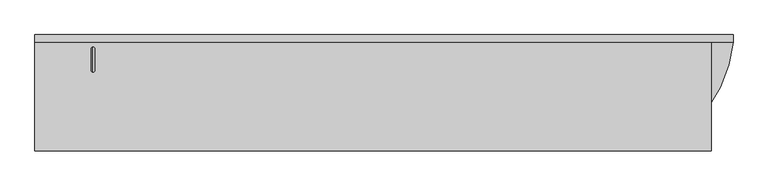
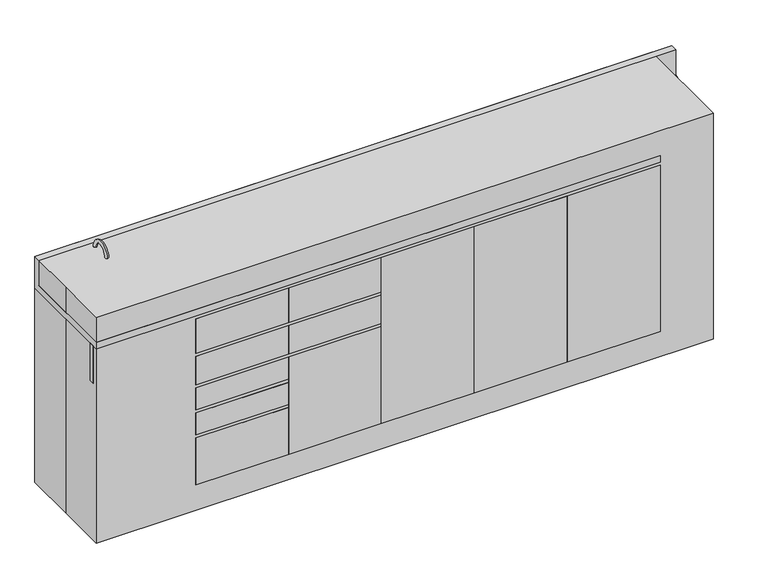
"""IFC4 building model written with IfcOpenShell, lengths in millimetres: proxy geometry, D0680 - Console, Accessory-Side, Dental Operatory-south sink-rounded : U0026 - Cabinet, Dental, Doctor's, Prosthodontic 2."""

import ifcopenshell
import ifcopenshell.guid

model = None  # the IFC model being written
_history = None  # IfcOwnerHistory: only IFC2X3 demands one
_inside = {}  # id of a spatial element -> (the spatial element, [elements in it])
_under = {}  # id of a project, library or spatial element -> (it, [spatial elements below it])
_declared = {}  # id of a project -> (the project, [libraries it declares])
_typed = {}  # id of a type object -> (the type object, [elements of that type])
_made_of = {}  # id of a material, layer set ... -> (it, [elements and type objects made of it])


def new_model(schema):
    """Start an empty IFC model of exactly this schema.

    Asked for "IFC4X3", IfcOpenShell would pick the latest addendum, in which some entities
    have other attributes; the version numbers below select the first issue.
    IFC2X3 requires an IfcOwnerHistory on every rooted entity: one is made here for all.
    """
    global model, _history
    if schema == "IFC4X3":
        model = ifcopenshell.file(schema_version=(4, 3, 0, 0))
    else:
        model = ifcopenshell.file(schema=schema)
    _inside.clear()
    _under.clear()
    _declared.clear()
    _typed.clear()
    _made_of.clear()
    _history = None
    if model.schema == "IFC2X3":
        org = make("IfcOrganization", Name="unknown")
        user = make(
            "IfcPersonAndOrganization",
            ThePerson=make("IfcPerson", FamilyName="unknown"),
            TheOrganization=org,
        )
        app = make(
            "IfcApplication",
            ApplicationDeveloper=org,
            Version="unknown",
            ApplicationFullName="unknown",
            ApplicationIdentifier="unknown",
        )
        _history = make(
            "IfcOwnerHistory",
            OwningUser=user,
            OwningApplication=app,
            ChangeAction="ADDED",
            CreationDate=0,
        )
    return model


def make(cls, **values):
    """One entity of the class cls with the attributes given. An attribute that is None is left unset."""
    return model.create_entity(
        cls, **{name: value for name, value in values.items() if value is not None}
    )


def rooted(cls, **values):
    """An entity with a GlobalId (a new one), such as an element, a storey or a relation."""
    return make(cls, GlobalId=ifcopenshell.guid.new(), OwnerHistory=_history, **values)


def si_unit(unit_type, name, prefix=None):
    """IfcSIUnit, for example si_unit("LENGTHUNIT", "METRE", prefix="MILLI")."""
    return make("IfcSIUnit", UnitType=unit_type, Prefix=prefix, Name=name)


def assignment(units):
    """IfcUnitAssignment: the units of a project."""
    return None if units is None else make("IfcUnitAssignment", Units=units)


def point(xyz):
    """IfcCartesianPoint."""
    return None if xyz is None else make("IfcCartesianPoint", Coordinates=xyz)


def direction(xyz):
    """IfcDirection."""
    return None if xyz is None else make("IfcDirection", DirectionRatios=xyz)


def frame(location, z_axis=None, x_axis=None):
    """IfcAxis2Placement3D, a coordinate frame: its origin and axes. An axis left out is left unset."""
    return make(
        "IfcAxis2Placement3D",
        Location=point(location),
        Axis=direction(z_axis),
        RefDirection=direction(x_axis),
    )


def frame_2d(location, x_axis=None):
    """IfcAxis2Placement2D, a coordinate frame in the plane: its origin and x axis."""
    return make(
        "IfcAxis2Placement2D", Location=point(location), RefDirection=direction(x_axis)
    )


def origin():
    """The frame at (0, 0, 0) with its axes left unset."""
    return frame((0.0, 0.0, 0.0))


def origin_with_axes():
    """The frame at (0, 0, 0) with the z axis (0, 0, 1) and the x axis (1, 0, 0) written out."""
    return frame((0.0, 0.0, 0.0), z_axis=(0.0, 0.0, 1.0), x_axis=(1.0, 0.0, 0.0))


def place(relative_to, where):
    """IfcLocalPlacement: puts the frame where relative to a parent placement (None: the world)."""
    return make(
        "IfcLocalPlacement", PlacementRelTo=relative_to, RelativePlacement=where
    )


def context(
    kind, dimensions, precision=None, world=None, true_north=None, identifier=None
):
    """IfcGeometricRepresentationContext, for example the 3D "Model" context."""
    return make(
        "IfcGeometricRepresentationContext",
        ContextIdentifier=identifier,
        ContextType=kind,
        CoordinateSpaceDimension=dimensions,
        Precision=precision,
        WorldCoordinateSystem=world,
        TrueNorth=true_north,
    )


def project(units=None, contexts=None):
    """IfcProject with its units and contexts."""
    return rooted(
        "IfcProject",
        Name="project",
        RepresentationContexts=contexts,
        UnitsInContext=assignment(units),
    )


def spatial(cls, under=None, at=None, **own):
    """A site, building, storey or space (cls), placed at a placement, below another one or the project."""
    s = rooted(cls, ObjectPlacement=at, **own)
    if under is not None:
        _under.setdefault(under.id(), (under, []))[1].append(s)
    return s


def polyline(points):
    """IfcPolyline through the points."""
    return make("IfcPolyline", Points=[point(p) for p in points])


def circle_curve(where, radius):
    """IfcCircle in the frame where."""
    return make("IfcCircle", Position=where, Radius=radius)


def ellipse_curve(where, semi_axis1, semi_axis2):
    """IfcEllipse in the frame where."""
    return make(
        "IfcEllipse", Position=where, SemiAxis1=semi_axis1, SemiAxis2=semi_axis2
    )


def trimmed(basis, trim1, trim2, sense, master):
    """IfcTrimmedCurve: the piece of a basis curve between two trims."""
    return make(
        "IfcTrimmedCurve",
        BasisCurve=basis,
        Trim1=trim1,
        Trim2=trim2,
        SenseAgreement=sense,
        MasterRepresentation=master,
    )


def segment(curve, same_sense, transition):
    """IfcCompositeCurveSegment."""
    return make(
        "IfcCompositeCurveSegment",
        Transition=transition,
        SameSense=same_sense,
        ParentCurve=curve,
    )


def composite_curve(segments, self_intersect=None):
    """IfcCompositeCurve: segments joined end to end."""
    return make("IfcCompositeCurve", Segments=segments, SelfIntersect=self_intersect)


def outline(outer, holes=None, kind="AREA"):
    """IfcArbitraryClosedProfileDef: a profile drawn as a closed curve; with holes, ...WithVoids."""
    if holes is None:
        return make("IfcArbitraryClosedProfileDef", ProfileType=kind, OuterCurve=outer)
    return make(
        "IfcArbitraryProfileDefWithVoids",
        ProfileType=kind,
        OuterCurve=outer,
        InnerCurves=holes,
    )


def extrude(swept, where, along, depth):
    """IfcExtrudedAreaSolid: the profile swept, set in the frame where, extruded along a direction by depth."""
    return make(
        "IfcExtrudedAreaSolid",
        SweptArea=swept,
        Position=where,
        ExtrudedDirection=direction(along),
        Depth=depth,
    )


def shape(context_of_items, identifier, shape_type, items):
    """IfcShapeRepresentation: the items that make up one representation, for example the "Body"."""
    return make(
        "IfcShapeRepresentation",
        ContextOfItems=context_of_items,
        RepresentationIdentifier=identifier,
        RepresentationType=shape_type,
        Items=items,
    )


def source(mapping_origin, context_of_items, identifier, shape_type, items):
    """IfcRepresentationMap: a shape defined once, which mapped items show again and again."""
    return make(
        "IfcRepresentationMap",
        MappingOrigin=mapping_origin,
        MappedRepresentation=shape(context_of_items, identifier, shape_type, items),
    )


def transform(
    local_origin,
    x_axis=None,
    y_axis=None,
    z_axis=None,
    scale=None,
    scale2=None,
    scale3=None,
    uniform=True,
):
    """IfcCartesianTransformationOperator3D, or its non-uniform kind. x_axis, y_axis, z_axis: its Axis1, 2, 3."""
    if uniform:
        return make(
            "IfcCartesianTransformationOperator3D",
            Axis1=direction(x_axis),
            Axis2=direction(y_axis),
            LocalOrigin=point(local_origin),
            Scale=scale,
            Axis3=direction(z_axis),
        )
    return make(
        "IfcCartesianTransformationOperator3DnonUniform",
        Axis1=direction(x_axis),
        Axis2=direction(y_axis),
        LocalOrigin=point(local_origin),
        Scale=scale,
        Axis3=direction(z_axis),
        Scale2=scale2,
        Scale3=scale3,
    )


def mapped(mapping_source, mapping_target):
    """IfcMappedItem: shows the shape of a source again, moved by a transform."""
    return make(
        "IfcMappedItem", MappingSource=mapping_source, MappingTarget=mapping_target
    )


def made_of(thing, what):
    """Note that an element or type object is made of a material, layer set ...; save() writes the relation."""
    if what is not None:
        _made_of.setdefault(what.id(), (what, []))[1].append(thing)
    return thing


def element(
    cls,
    number,
    at=None,
    inside=None,
    cuts=None,
    type_object=None,
    material=None,
    context=None,
    identifier="Body",
    shape_type=None,
    held_by="IfcProductDefinitionShape",
    body=None,
    shapes=None,
    **own,
):
    """One element of the class cls, such as IfcWall. Its Tag is "e" and its number.

    at: its placement. inside: the storey or other place that contains it. cuts: it is an
    opening in that element (IfcRelVoidsElement). A single representation is given by context,
    identifier, shape_type and body (its items); several are given by shapes. held_by: the class
    of the entity that holds the representations. save() writes the other relations.
    """
    e = rooted(cls, Tag="e%d" % number, ObjectPlacement=at, **own)
    if body is not None:
        shapes = [shape(context, identifier, shape_type, body)]
    if shapes is not None:
        e.Representation = make(held_by, Representations=shapes)
    if inside is not None:
        _inside.setdefault(inside.id(), (inside, []))[1].append(e)
    if cuts is not None:
        rooted(
            "IfcRelVoidsElement", RelatingBuildingElement=cuts, RelatedOpeningElement=e
        )
    if type_object is not None:
        _typed.setdefault(type_object.id(), (type_object, []))[1].append(e)
    return made_of(e, material)


def aggregate(whole, parts):
    """IfcRelAggregates: a whole, such as a stair, and the parts it consists of."""
    return rooted("IfcRelAggregates", RelatingObject=whole, RelatedObjects=parts)


def save(model, path):
    """Write the relations noted so far, then the file.

    IfcRelAggregates (storeys below a building ...), IfcRelContainedInSpatialStructure (elements
    in a storey), IfcRelDefinesByType, IfcRelAssociatesMaterial and IfcRelDeclares: one each for
    every whole, place, type object, material and project.
    """
    for whole, parts in _under.values():
        aggregate(whole, parts)
    for where, things in _inside.values():
        rooted(
            "IfcRelContainedInSpatialStructure",
            RelatedElements=things,
            RelatingStructure=where,
        )
    for kind, things in _typed.values():
        rooted("IfcRelDefinesByType", RelatedObjects=things, RelatingType=kind)
    for what, things in _made_of.values():
        rooted("IfcRelAssociatesMaterial", RelatedObjects=things, RelatingMaterial=what)
    for by, libraries in _declared.values():
        rooted("IfcRelDeclares", RelatingContext=by, RelatedDefinitions=libraries)
    model.write(path)


def plane_surface(at):
    """IfcPlane: the flat surface through the origin of the frame at, square to its z axis."""
    return make("IfcPlane", Position=at)


def cylinder_surface(at, radius):
    """IfcCylindricalSurface: all points at the distance radius from the z axis of the frame at."""
    return make("IfcCylindricalSurface", Position=at, Radius=radius)


def revolved_surface(curve, axis_point, axis_direction):
    """IfcSurfaceOfRevolution: the curve turned about the line through axis_point along axis_direction."""
    return make(
        "IfcSurfaceOfRevolution",
        SweptCurve=make("IfcArbitraryOpenProfileDef", ProfileType="CURVE", Curve=curve),
        AxisPosition=make("IfcAxis1Placement", Location=point(axis_point), Axis=direction(axis_direction)),
    )


def advanced_brep(points, edges, surfaces, faces):
    """IfcAdvancedBrep: a solid bounded by faces that lie on surfaces and meet in shared edges.

    An edge is (start, end): straight between two places in points (the first is 0);
    or (start, end, curve); or (start, end, curve, False) where it runs against its curve.
    A face is (place in surfaces, loops), or (place, loops, False) where it looks against
    its surface's normal. A loop lists edges by number (the first is 1), with a minus sign
    where the edge is run from its end to its start. The first loop is the outer one.
    """
    corners = [point(p) for p in points]
    vertices = [make("IfcVertexPoint", VertexGeometry=c) for c in corners]
    made = []
    for start, end, *more in edges:
        made.append(
            make(
                "IfcEdgeCurve",
                EdgeStart=vertices[start],
                EdgeEnd=vertices[end],
                EdgeGeometry=more[0] if more else make("IfcPolyline", Points=[corners[start], corners[end]]),
                SameSense=more[1] if len(more) > 1 else True,
            )
        )
    hull = []
    for where, loops, *sense in faces:
        bounds = []
        for j, loop in enumerate(loops):
            ring = [make("IfcOrientedEdge", EdgeElement=made[abs(k) - 1], Orientation=k > 0) for k in loop]
            bounds.append(
                make(
                    "IfcFaceOuterBound" if j == 0 else "IfcFaceBound",
                    Bound=make("IfcEdgeLoop", EdgeList=ring),
                    Orientation=True,
                )
            )
        hull.append(make("IfcAdvancedFace", Bounds=bounds, FaceSurface=surfaces[where], SameSense=sense[0] if sense else True))
    return make("IfcAdvancedBrep", Outer=make("IfcClosedShell", CfsFaces=hull))


def specialty_equipment_783713db(model_context):
    return source(origin(), model_context, "Body", "SolidModel", [
        advanced_brep(
        [(-1014.0443585, -165.0080446, 787.3899582), (-1014.0443585, 139.7919554, 787.3899582), (-1014.0443585, 128.6794554, 787.3899582), (-1014.0443585, -153.8955446, 787.3899582), (-1014.0443585, 127.0919554, 785.8024582), (-1014.0443585, -152.3080446, 785.8024582), (-1014.0443585, 127.0919554, 730.25), (-1014.0443585, -152.3080446, 730.25), (-1014.0443585, -101.5080446, 679.45), (-1014.0443585, 76.2919554, 679.45), (-1014.0443585, -0.1899284, 679.45), (-1003.5461263, -12.6976148, 679.45), (-1014.0443585, -25.2053012, 679.45), (-1028.9461263, -12.6976148, 679.45), (-1014.0443585, -158.6580446, 676.275), (-1014.0443585, 133.4419554, 676.275), (-1014.0443585, 133.4419554, 784.0168572), (-1014.0443585, -158.6580446, 784.0168572), (-1014.0443585, 139.7919554, 784.0168572), (-1014.0443585, -165.0080446, 784.0168572), (-1014.0443585, -25.2053012, 676.275), (-1003.5461263, -12.6976148, 676.275), (-1014.0443585, -0.1899284, 676.275), (-1028.9461263, -12.6976148, 676.275)],
        [
            (0, 1, circle_curve(frame((-1014.0443585, -12.6080446, 787.3899582), z_axis=(0.0, 0.0, 1.0), x_axis=(0.0, 1.0, 0.0)), 152.4)),
            (1, 2),
            (2, 3, circle_curve(frame((-1014.0443585, -12.6080446, 787.3899582), z_axis=(0.0, 0.0, -1.0), x_axis=(0.0, 1.0, 0.0)), 141.2875)),
            (3, 0),
            (1, 0, circle_curve(frame((-1014.0443585, -12.6080446, 787.3899582), z_axis=(0.0, 0.0, 1.0), x_axis=(0.0, 1.0, 0.0)), 152.4)),
            (3, 2, circle_curve(frame((-1014.0443585, -12.6080446, 787.3899582), z_axis=(0.0, 0.0, -1.0), x_axis=(0.0, 1.0, 0.0)), 141.2875)),
            (2, 4, circle_curve(frame((-1014.0443585, 128.6794554, 785.8024582), z_axis=(1.0, 0.0, 0.0), x_axis=(0.0, 1.0, 0.0)), 1.5875)),
            (4, 5, circle_curve(frame((-1014.0443585, -12.6080446, 785.8024582), z_axis=(0.0, 0.0, -1.0), x_axis=(0.0, 1.0, 0.0)), 139.7)),
            (5, 3, circle_curve(frame((-1014.0443585, -153.8955446, 785.8024582), z_axis=(1.0, 0.0, 0.0), x_axis=(0.0, -1.0, 0.0)), 1.5875)),
            (5, 4, circle_curve(frame((-1014.0443585, -12.6080446, 785.8024582), z_axis=(0.0, 0.0, -1.0), x_axis=(0.0, 1.0, 0.0)), 139.7)),
            (4, 6),
            (6, 7, circle_curve(frame((-1014.0443585, -12.6080446, 730.25), z_axis=(0.0, 0.0, -1.0), x_axis=(0.0, 1.0, 0.0)), 139.7)),
            (7, 5),
            (7, 6, circle_curve(frame((-1014.0443585, -12.6080446, 730.25), z_axis=(0.0, 0.0, -1.0), x_axis=(0.0, 1.0, 0.0)), 139.7)),
            (8, 9, circle_curve(frame((-1014.0443585, -12.6080446, 679.45), z_axis=(0.0, 0.0, 1.0), x_axis=(0.0, 1.0, 0.0)), 88.9)),
            (9, 10),
            (10, 11, circle_curve(frame((-1016.2461263, -12.6976148, 679.45), z_axis=(0.0, 0.0, -1.0), x_axis=(-1.0, 0.0, 0.0)), 12.7)),
            (11, 12, circle_curve(frame((-1016.2461263, -12.6976148, 679.45), z_axis=(0.0, 0.0, -1.0), x_axis=(-1.0, 0.0, 0.0)), 12.7)),
            (12, 8),
            (9, 8, circle_curve(frame((-1014.0443585, -12.6080446, 679.45), z_axis=(0.0, 0.0, 1.0), x_axis=(0.0, 1.0, 0.0)), 88.9)),
            (12, 13, circle_curve(frame((-1016.2461263, -12.6976148, 679.45), z_axis=(0.0, 0.0, -1.0), x_axis=(-1.0, 0.0, 0.0)), 12.7)),
            (13, 10, circle_curve(frame((-1016.2461263, -12.6976148, 679.45), z_axis=(0.0, 0.0, -1.0), x_axis=(-1.0, 0.0, 0.0)), 12.7)),
            (14, 15, circle_curve(frame((-1014.0443585, -12.6080446, 676.275), z_axis=(0.0, 0.0, 1.0), x_axis=(0.0, 1.0, 0.0)), 146.05)),
            (15, 16),
            (16, 17, circle_curve(frame((-1014.0443585, -12.6080446, 784.0168572), z_axis=(0.0, 0.0, -1.0), x_axis=(0.0, 1.0, 0.0)), 146.05)),
            (17, 14),
            (15, 14, circle_curve(frame((-1014.0443585, -12.6080446, 676.275), z_axis=(0.0, 0.0, 1.0), x_axis=(0.0, 1.0, 0.0)), 146.05)),
            (17, 16, circle_curve(frame((-1014.0443585, -12.6080446, 784.0168572), z_axis=(0.0, 0.0, -1.0), x_axis=(0.0, 1.0, 0.0)), 146.05)),
            (16, 18),
            (18, 19, circle_curve(frame((-1014.0443585, -12.6080446, 784.0168572), z_axis=(0.0, 0.0, -1.0), x_axis=(0.0, 1.0, 0.0)), 152.4)),
            (19, 17),
            (19, 18, circle_curve(frame((-1014.0443585, -12.6080446, 784.0168572), z_axis=(0.0, 0.0, -1.0), x_axis=(0.0, 1.0, 0.0)), 152.4)),
            (0, 19),
            (18, 1),
            (14, 20),
            (20, 21, circle_curve(frame((-1016.2461263, -12.6976148, 676.275), z_axis=(0.0, 0.0, 1.0), x_axis=(-1.0, 0.0, 0.0)), 12.7)),
            (21, 22, circle_curve(frame((-1016.2461263, -12.6976148, 676.275), z_axis=(0.0, 0.0, 1.0), x_axis=(-1.0, 0.0, 0.0)), 12.7)),
            (22, 15),
            (22, 23, circle_curve(frame((-1016.2461263, -12.6976148, 676.275), z_axis=(0.0, 0.0, 1.0), x_axis=(-1.0, 0.0, 0.0)), 12.7)),
            (23, 20, circle_curve(frame((-1016.2461263, -12.6976148, 676.275), z_axis=(0.0, 0.0, 1.0), x_axis=(-1.0, 0.0, 0.0)), 12.7)),
            (6, 9, circle_curve(frame((-1014.0443585, 76.2919554, 730.25), z_axis=(-1.0, 0.0, 0.0), x_axis=(0.0, 1.0, 0.0)), 50.8)),
            (8, 7, circle_curve(frame((-1014.0443585, -101.5080446, 730.25), z_axis=(-1.0, 0.0, 0.0), x_axis=(0.0, -1.0, 0.0)), 50.8)),
            (23, 13),
            (11, 21),
        ],
        [
            plane_surface(frame((-1014.0443585, -12.6080446, 787.3899582), z_axis=(0.0, 0.0, 1.0), x_axis=(0.0, 1.0, 0.0))),
            revolved_surface(trimmed(ellipse_curve(frame((-1014.0443585, 128.6794554, 785.8024582), z_axis=(-1.0, 0.0, 0.0), x_axis=(0.0, 1.0, 0.0)), 1.5875, 1.5875), [point((-1014.0443585, 127.0919554, 785.8024582))], [point((-1014.0443585, 128.6794554, 787.3899582))], True, "CARTESIAN"), (-1014.0443585, -12.6080446, 787.4), (0.0, 0.0, -1.0)),
            revolved_surface(polyline([(-1014.0443585, 127.09195539999999, 730.25), (-1014.0443585, 127.09195539999999, 785.8024582)]), (-1014.0443585, -12.6080446, 787.4), (0.0, 0.0, -1.0)),
            plane_surface(frame((-1014.0443585, -12.6080446, 679.45), z_axis=(0.0, 0.0, 1.0), x_axis=(0.0, 1.0, 0.0))),
            cylinder_surface(frame((-1014.0443585, -12.6080446, 787.4), z_axis=(0.0, 0.0, -1.0), x_axis=(0.0, 1.0, 0.0)), 146.05),
            plane_surface(frame((-1014.0443585, -12.6080446, 784.0168572), z_axis=(0.0, 0.0, -1.0), x_axis=(0.0, 1.0, 0.0))),
            cylinder_surface(frame((-1014.0443585, -12.6080446, 787.4), z_axis=(0.0, 0.0, -1.0), x_axis=(0.0, 1.0, 0.0)), 152.4),
            plane_surface(frame((-1014.0443585, -12.6080446, 676.275), z_axis=(0.0, 0.0, -1.0), x_axis=(0.0, 1.0, 0.0))),
            revolved_surface(trimmed(ellipse_curve(frame((-1014.0443585, 76.2919554, 730.25), z_axis=(1.0, 0.0, 0.0), x_axis=(0.0, 1.0, 0.0)), 50.8, 50.8), [point((-1014.0443585, 76.2919554, 679.45))], [point((-1014.0443585, 127.0919554, 730.25))], True, "CARTESIAN"), (-1014.0443585, -12.6080446, 787.4), (0.0, 0.0, -1.0)),
            revolved_surface(polyline([(-1028.9461263, -12.6976148, 679.45), (-1028.9461263, -12.6976148, 676.275)]), (-1016.2461263, -12.6976148, 673.1), (0.0, 0.0, 1.0)),
        ],
        [
            (0, [[1, 2, 3, 4]]),
            (0, [[-2, 5, -4, 6]]),
            (1, [[-3, 7, 8, 9]]),
            (1, [[-6, -9, 10, -7]]),
            (2, [[-8, 11, 12, 13]]),
            (2, [[-10, -13, 14, -11]]),
            (3, [[15, 16, 17, 18, 19]]),
            (3, [[20, -19, 21, 22, -16]]),
            (4, [[23, 24, 25, 26]]),
            (4, [[-24, 27, -26, 28]]),
            (5, [[-25, 29, 30, 31]]),
            (5, [[-28, -31, 32, -29]]),
            (6, [[-1, 33, -30, 34]]),
            (6, [[-5, -34, -32, -33]]),
            (7, [[-23, 35, 36, 37, 38]]),
            (7, [[-27, -38, 39, 40, -35]]),
            (8, [[-12, 41, -15, 42]]),
            (8, [[-14, -42, -20, -41]]),
            (9, [[43, -21, -18, 44, -36, -40]]),
            (9, [[-43, -39, -37, -44, -17, -22]]),
        ],
    ),
        extrude(outline(polyline([(-1219.2, -184.15), (-1219.2, -165.1), (-850.9, -165.1), (-850.9, -184.15), (-1219.2, -184.15)])), frame((0.0, 0.0, 635.0), z_axis=(0.0, 0.0, 1.0), x_axis=(1.0, 0.0, 0.0)), (0.0, 0.0, 1.0), 152.4),
        extrude(outline(polyline([(-184.15, 101.6), (-203.2, 101.6), (-203.2, 774.4822891), (-193.675, 774.4822891), (-193.675, 787.2846899), (-184.15, 787.2846899), (-184.15, 101.6)])), frame((584.2, 0.0, 0.0), z_axis=(1.0, 0.0, 0.0), x_axis=(0.0, 1.0, 0.0)), (0.0, 0.0, 1.0), 355.6),
        extrude(outline(polyline([(-184.15, 101.6), (-203.2, 101.6), (-203.2, 774.7), (-193.675, 774.7), (-193.675, 787.4), (-184.15, 787.4), (-184.15, 101.6)])), frame((228.6, 0.0, 0.0), z_axis=(1.0, 0.0, 0.0), x_axis=(0.0, 1.0, 0.0)), (0.0, 0.0, 1.0), 355.6),
        extrude(outline(polyline([(-184.15, 101.6), (-203.2, 101.6), (-203.2, 774.7), (-193.675, 774.7), (-193.675, 787.4), (-184.15, 787.4), (-184.15, 101.6)])), frame((-127.0, 0.0, 0.0), z_axis=(1.0, 0.0, 0.0), x_axis=(0.0, 1.0, 0.0)), (0.0, 0.0, 1.0), 355.6),
        extrude(outline(polyline([(-193.675, 774.7), (-193.675, 787.4), (-184.15, 787.4), (-184.15, 635.0), (-203.2, 635.0), (-203.2, 774.7), (-193.675, 774.7)])), frame((-482.6, 0.0, 0.0), z_axis=(1.0, 0.0, 0.0), x_axis=(0.0, 1.0, 0.0)), (0.0, 0.0, 1.0), 355.6),
        extrude(outline(polyline([(-193.675, 622.9156171), (-193.675, 635.0), (-184.15, 635.0), (-184.15, 508.0524006), (-203.2, 508.0524006), (-203.2, 622.9156171), (-193.675, 622.9156171)])), frame((-482.6, 0.0, 0.0), z_axis=(1.0, 0.0, 0.0), x_axis=(0.0, 1.0, 0.0)), (0.0, 0.0, 1.0), 355.6),
        extrude(outline(polyline([(-193.675, 495.2120809), (-193.675, 508.0517033), (-184.15, 508.0517033), (-184.15, 101.6), (-203.2, 101.6), (-203.2, 495.2120809), (-193.675, 495.2120809)])), frame((-482.6, 0.0, 0.0), z_axis=(1.0, 0.0, 0.0), x_axis=(0.0, 1.0, 0.0)), (0.0, 0.0, 1.0), 355.6),
        extrude(outline(composite_curve([segment(trimmed(circle_curve(frame_2d((-1053.7479232, 156.0133962)), 12.7), [point((-1041.0479232, 156.0133962))], [point((-1066.4479232, 156.0133962))], False, "CARTESIAN"), True, "CONTINUOUS"), segment(trimmed(circle_curve(frame_2d((-1053.7479232, 156.0133962)), 12.7), [point((-1066.4479232, 156.0133962))], [point((-1041.0479232, 156.0133962))], False, "CARTESIAN"), True, "CONTINUOUS")], self_intersect=False)), frame((0.0, 0.0, 812.8), z_axis=(0.0, 0.0, 1.0), x_axis=(1.0, 0.0, 0.0)), (0.0, 0.0, 1.0), 31.75),
        extrude(outline(composite_curve([segment(trimmed(circle_curve(frame_2d((-980.5384765, 156.0133962)), 12.7), [point((-967.8384765, 156.0133962))], [point((-993.2384765, 156.0133962))], False, "CARTESIAN"), True, "CONTINUOUS"), segment(trimmed(circle_curve(frame_2d((-980.5384765, 156.0133962)), 12.7), [point((-993.2384765, 156.0133962))], [point((-967.8384765, 156.0133962))], False, "CARTESIAN"), True, "CONTINUOUS")], self_intersect=False)), frame((0.0, 0.0, 812.8), z_axis=(0.0, 0.0, 1.0), x_axis=(1.0, 0.0, 0.0)), (0.0, 0.0, 1.0), 31.75),
        advanced_brep(
        [(-1016.415785, 148.0147812, 812.8), (-1016.415785, 160.7147812, 812.8), (-1016.415785, 160.7147812, 914.4), (-1016.415785, 148.0147812, 914.4), (-1016.415785, 84.5147812, 914.4), (-1016.415785, 71.8147812, 914.4)],
        [
            (0, 1, circle_curve(frame((-1016.415785, 154.3647812, 812.8), z_axis=(0.0, 0.0, -1.0), x_axis=(0.0, 1.0, 0.0)), 6.35)),
            (1, 0, circle_curve(frame((-1016.415785, 154.3647812, 812.8), z_axis=(0.0, 0.0, -1.0), x_axis=(0.0, 1.0, 0.0)), 6.35)),
            (1, 2),
            (2, 3, circle_curve(frame((-1016.415785, 154.3647812, 914.4), z_axis=(0.0, 0.0, -1.0), x_axis=(0.0, 1.0, 0.0)), 6.35)),
            (3, 0),
            (3, 2, circle_curve(frame((-1016.415785, 154.3647812, 914.4), z_axis=(0.0, 0.0, -1.0), x_axis=(0.0, 1.0, 0.0)), 6.35)),
            (4, 5, circle_curve(frame((-1016.415785, 78.1647812, 914.4), z_axis=(0.0, 0.0, -1.0), x_axis=(0.0, -1.0, 0.0)), 6.35)),
            (5, 4, circle_curve(frame((-1016.415785, 78.1647812, 914.4), z_axis=(0.0, 0.0, -1.0), x_axis=(0.0, -1.0, 0.0)), 6.35)),
            (4, 3, circle_curve(frame((-1016.415785, 116.2647812, 914.4), z_axis=(-1.0, 0.0, 0.0), x_axis=(0.0, 1.0, 0.0)), 31.75)),
            (2, 5, circle_curve(frame((-1016.415785, 116.2647812, 914.4), z_axis=(1.0, 0.0, 0.0), x_axis=(0.0, 1.0, 0.0)), 44.45)),
        ],
        [
            plane_surface(frame((-1104.9, 154.3647812, 812.8), z_axis=(0.0, 0.0, -1.0), x_axis=(-1.0, 0.0, 0.0))),
            cylinder_surface(frame((-1016.415785, 154.3647812, 812.8), z_axis=(0.0, 0.0, -1.0), x_axis=(0.0, 1.0, 0.0)), 6.35),
            plane_surface(frame((-1104.9, 78.1647812, 914.4), z_axis=(0.0, 0.0, -1.0), x_axis=(-1.0, 0.0, 0.0))),
            revolved_surface(trimmed(ellipse_curve(frame((-1016.415785, 154.3647812, 914.4), z_axis=(0.0, 0.0, -1.0), x_axis=(0.0, 1.0, 0.0)), 6.35, 6.35), [point((-1016.415785, 160.7147812, 914.4))], [point((-1016.415785, 148.0147812, 914.4))], True, "CARTESIAN"), (-1104.9, 116.2647812, 914.4), (1.0, 0.0, 0.0)),
            revolved_surface(trimmed(ellipse_curve(frame((-1016.415785, 154.3647812, 914.4), z_axis=(0.0, 0.0, -1.0), x_axis=(0.0, 1.0, 0.0)), 6.35, 6.35), [point((-1016.415785, 148.0147812, 914.4))], [point((-1016.415785, 160.7147812, 914.4))], True, "CARTESIAN"), (-1104.9, 116.2647812, 914.4), (1.0, 0.0, 0.0)),
        ],
        [
            (0, [[1, 2]]),
            (1, [[-2, 3, 4, 5]]),
            (1, [[-1, -5, 6, -3]]),
            (2, [[7, 8]]),
            (3, [[9, -4, 10, -7]]),
            (4, [[-10, -6, -9, -8]]),
        ],
    ),
        extrude(outline(polyline([(-193.675, 774.7), (-193.675, 787.4), (-184.15, 787.4), (-184.15, 635.0), (-203.2, 635.0), (-203.2, 774.7), (-193.675, 774.7)])), frame((-838.2, 0.0, 0.0), z_axis=(1.0, 0.0, 0.0), x_axis=(0.0, 1.0, 0.0)), (0.0, 0.0, 1.0), 355.6),
        extrude(outline(polyline([(-193.675, 622.9156171), (-193.675, 635.0), (-184.15, 635.0), (-184.15, 508.0), (-203.2, 508.0), (-203.2, 622.9156171), (-193.675, 622.9156171)])), frame((-838.2, 0.0, 0.0), z_axis=(1.0, 0.0, 0.0), x_axis=(0.0, 1.0, 0.0)), (0.0, 0.0, 1.0), 355.6),
        extrude(outline(polyline([(-193.675, 495.3), (-193.675, 508.0), (-184.15, 508.0), (-184.15, 406.4), (-203.2, 406.4), (-203.2, 495.3), (-193.675, 495.3)])), frame((-838.2, 0.0, 0.0), z_axis=(1.0, 0.0, 0.0), x_axis=(0.0, 1.0, 0.0)), (0.0, 0.0, 1.0), 355.6),
        extrude(outline(polyline([(-193.675, 393.7), (-193.675, 406.4), (-184.15, 406.4), (-184.15, 304.8), (-203.2, 304.8), (-203.2, 393.7), (-193.675, 393.7)])), frame((-838.2, 0.0, 0.0), z_axis=(1.0, 0.0, 0.0), x_axis=(0.0, 1.0, 0.0)), (0.0, 0.0, 1.0), 355.6),
        extrude(outline(polyline([(-193.675, 292.1), (-193.675, 304.8), (-184.15, 304.8), (-184.15, 101.6), (-203.2, 101.6), (-203.2, 292.1), (-193.675, 292.1)])), frame((-838.2, 0.0, 0.0), z_axis=(1.0, 0.0, 0.0), x_axis=(0.0, 1.0, 0.0)), (0.0, 0.0, 1.0), 355.6),
        advanced_brep(
        [(-1219.2, 177.8, 914.4), (-1219.2, 203.2, 914.4), (-1219.2, 203.2, 787.4), (-1219.2, -203.2, 787.4), (-1219.2, -203.2, 812.8), (-1219.2, 177.8, 812.8), (1219.2, 177.8, 812.8), (1219.2, 177.8, 863.6), (1219.2, 177.8, 914.4), (939.8, -203.2, 812.8), (-874.2071906, -12.5959993, 812.8), (-1153.6071906, -12.5959993, 812.8), (939.8, -203.2, 787.4), (1219.2, 203.2, 787.4), (1219.2, 177.8, 787.4), (-1153.6071906, -12.5959993, 787.4), (-874.2071906, -12.5959993, 787.4), (1219.2, 203.2, 914.4)],
        [
            (0, 1),
            (1, 2),
            (2, 3),
            (3, 4),
            (4, 5),
            (5, 0),
            (5, 6),
            (6, 7),
            (7, 8),
            (8, 0),
            (4, 9),
            (9, 6, circle_curve(frame((763.8405952, 218.7835635, 812.8), z_axis=(0.0, 0.0, 1.0), x_axis=(1.0, 0.0, 0.0)), 457.2)),
            (10, 11, circle_curve(frame((-1013.9071906, -12.5959993, 812.8), z_axis=(0.0, 0.0, -1.0), x_axis=(-1.0, 0.0, 0.0)), 139.7)),
            (11, 10, circle_curve(frame((-1013.9071906, -12.5959993, 812.8), z_axis=(0.0, 0.0, -1.0), x_axis=(-1.0, 0.0, 0.0)), 139.7)),
            (3, 12),
            (12, 9),
            (2, 13),
            (13, 14),
            (14, 12, circle_curve(frame((763.8405952, 218.7835635, 787.4), z_axis=(0.0, 0.0, -1.0), x_axis=(1.0, 0.0, 0.0)), 457.2)),
            (15, 16, circle_curve(frame((-1013.9071906, -12.5959993, 787.4), z_axis=(0.0, 0.0, 1.0), x_axis=(-1.0, 0.0, 0.0)), 139.7)),
            (16, 15, circle_curve(frame((-1013.9071906, -12.5959993, 787.4), z_axis=(0.0, 0.0, 1.0), x_axis=(-1.0, 0.0, 0.0)), 139.7)),
            (17, 13),
            (1, 17),
            (8, 17),
            (15, 11),
            (10, 16),
            (6, 14),
        ],
        [
            plane_surface(frame((-1219.2, 177.8, 812.8), z_axis=(-1.0, 0.0, 0.0), x_axis=(0.0, 0.0, 1.0))),
            plane_surface(frame((1219.2, 177.8, 914.4), z_axis=(0.0, -1.0, 0.0), x_axis=(-1.0, 0.0, 0.0))),
            plane_surface(frame((1219.2, 177.8, 812.8), z_axis=(0.0, 0.0, 1.0), x_axis=(-1.0, 0.0, 0.0))),
            plane_surface(frame((1219.2, -203.2, 812.8), z_axis=(0.0, -1.0, 0.0), x_axis=(-1.0, 0.0, 0.0))),
            plane_surface(frame((1219.2, -203.2, 787.4), z_axis=(0.0, 0.0, -1.0), x_axis=(-1.0, 0.0, 0.0))),
            plane_surface(frame((1219.2, 203.2, 787.4), z_axis=(0.0, 1.0, 0.0), x_axis=(-1.0, 0.0, 0.0))),
            plane_surface(frame((1219.2, 203.2, 914.4), z_axis=(0.0, 0.0, 1.0), x_axis=(-1.0, 0.0, 0.0))),
            revolved_surface(polyline([(-1153.6071906, -12.5959993, 812.8), (-1153.6071906, -12.5959993, 787.4)]), (-1013.9071906, -12.5959993, 768.35), (0.0, 0.0, 1.0)),
            plane_surface(frame((1219.2, 177.8, 812.8), z_axis=(1.0, 0.0, 0.0), x_axis=(0.0, 0.0, -1.0))),
            cylinder_surface(frame((763.8405952, 218.7835635, 736.6), z_axis=(0.0, 0.0, -1.0), x_axis=(1.0, 0.0, 0.0)), 457.2),
        ],
        [
            (0, [[1, 2, 3, 4, 5, 6]]),
            (1, [[-6, 7, 8, 9, 10]]),
            (2, [[-5, 11, 12, -7], [13, 14]]),
            (3, [[-4, 15, 16, -11]]),
            (4, [[-3, 17, 18, 19, -15], [20, 21]]),
            (5, [[22, -17, -2, 23]]),
            (6, [[24, -23, -1, -10]]),
            (7, [[25, -13, 26, -20]]),
            (7, [[-25, -21, -26, -14]]),
            (8, [[-22, -24, -9, -8, 27, -18]]),
            (9, [[-27, -12, -16, -19]]),
        ],
    ),
        extrude(outline(polyline([(-1219.2, 203.2), (1143.0, 203.2), (1143.0, -203.2), (-1219.2, -203.2), (-1219.2, 0.0), (-1219.2, 203.2)])), origin_with_axes(), (0.0, 0.0, 1.0), 914.4),
        extrude(outline(polyline([(184.15, 785.890324), (184.15, 0.0), (-165.1, 0.0), (-165.1, 101.6), (-184.15, 101.6), (-184.15, 785.890324), (184.15, 785.890324)])), frame((939.8, 0.0, 0.0), z_axis=(1.0, 0.0, 0.0), x_axis=(0.0, 1.0, 0.0)), (0.0, 0.0, 1.0), 12.7),
        extrude(outline(polyline([(1199.3554733, 184.15), (-850.9, 184.15), (-850.9, 203.2), (1199.3554733, 203.2), (1199.3554733, 184.15)])), origin_with_axes(), (0.0, 0.0, 1.0), 787.6898809),
        extrude(outline(polyline([(-117.475, 184.15), (-117.475, -184.15), (-136.525, -184.15), (-136.525, 184.15), (-117.475, 184.15)])), frame((0.0, 0.0, 120.7166954), z_axis=(0.0, 0.0, 1.0), x_axis=(1.0, 0.0, 0.0)), (0.0, 0.0, 1.0), 653.9833046),
        extrude(outline(polyline([(184.15, 787.4), (184.15, 0.0), (-165.1, 0.0), (-165.1, 101.6), (-184.15, 101.6), (-184.15, 787.4), (184.15, 787.4)])), frame((-850.9, 0.0, 0.0), z_axis=(1.0, 0.0, 0.0), x_axis=(0.0, 1.0, 0.0)), (0.0, 0.0, 1.0), 12.7),
        extrude(outline(polyline([(-473.075, 184.15), (-473.075, -184.15), (-492.125, -184.15), (-492.125, 184.15), (-473.075, 184.15)])), frame((0.0, 0.0, 120.7166954), z_axis=(0.0, 0.0, 1.0), x_axis=(1.0, 0.0, 0.0)), (0.0, 0.0, 1.0), 666.6833046),
        extrude(outline(polyline([(952.5, -184.15), (-850.9, -184.15), (-850.9, -165.1), (952.5, -165.1), (952.5, -184.15)])), origin_with_axes(), (0.0, 0.0, 1.0), 101.6),
        extrude(outline(polyline([(-838.2, 184.15), (939.8, 184.15), (939.8, -184.15), (-838.2, -184.15), (-838.2, 184.15)])), frame((0.0, 0.0, 101.6), z_axis=(0.0, 0.0, 1.0), x_axis=(1.0, 0.0, 0.0)), (0.0, 0.0, 1.0), 19.1166954),
    ])


if __name__ == "__main__":
    model = new_model("IFC4")
    model_context = context("Model", 3, world=origin())
    ifc_project = project(units=[si_unit("LENGTHUNIT", "METRE", prefix="MILLI")], contexts=[model_context])
    site = spatial("IfcSite", under=ifc_project)
    building = spatial("IfcBuilding", under=site)
    placement = place(None, origin())
    specialty_equipment_shape = specialty_equipment_783713db(model_context)
    element("IfcBuildingElementProxy", 1, Name="D0680 - Console, Accessory-Side, Dental Operatory-south sink-rounded : U0026 - Cabinet, Dental, Doctor's, Prosthodontic 2", ObjectType="D0680 - Console, Accessory-Side, Dental Operatory-south sink-rounded : U0026 - Cabinet, Dental, Doctor's, Prosthodontic 2", at=placement, inside=building, context=model_context, shape_type="MappedRepresentation", body=[
        mapped(specialty_equipment_shape, transform((0.0, 0.0, 0.0), x_axis=(1.0, 0.0, 0.0), y_axis=(0.0, 1.0, 0.0), z_axis=(0.0, 0.0, 1.0))),
    ])
    save(model, "model.ifc")

# Revit data of these elements
# Type "D0680 - Console, Accessory-Side, Dental Operatory-south sink-rounded : U0026 - Cabinet, Dental, Doctor's, Prosthodontic 2"
#   Watts2 = "0"
#   Watts1 = "120"
#   Unit_Issue = "EA"
#   UTIL_6_Misc = "-"
#   UTIL_5_NonMedGas = "-"
#   UTIL_4_MiscGas = "-"
#   UTIL_3_MedGas = "-"
#   UTIL_2_Elec = "A"
#   UTIL_1_WaterDrain = "D"
#   Nomenclature = "Console, Accessory/Side, Dental Operatory"
#   NSN = "6520"
#   Location [instance default] = ""
#   JSN = "D0680"
#   Fund_Source_VA = "-"
#   Fund_Source_Navy = "-"
#   Fund_Source_Army = "-"
#   Fund_Source_AF = "-"
#   ELEC_Volts2 = "0"
#   ELEC_Volts1 = "120"
#   ELEC_Phase2 = "0"
#   ELEC_Phase1 = "1"
#   ELEC_HertzSwitch = "0"
#   ELEC_HertzDependent = "-1"
#   ELEC_Hertz = "60"
#   ELEC_Amps2 = "0"
#   ELEC_Amps1 = "1"
#   DetailDescription = "An accessory or side console/cabinet approximately 60\" W x24\"D x 32\"H for use in a single chair dental operatory. The console may be a left or a right unit used for the dentist or the assistant depending configuration of the operatory. The unit may contain a sink component with waste drop, a round SS sink with faucet and soap dispenser, a solid surface counter top, a drawer storage module with writing surface and equipment drawers, a double door component with swing out shelves and a glove dispenser. Various combinations are available as well as different widths. Configuration of the unit, including whether the unit is right or left, to be determined at time of purchase."
#   CAT_VA = "A"
#   CAT_Navy = "A"
#   CAT_IHS = "-"
#   CAT_Army = "A"
#   CAT_AF = "A"
#   BTUperhour = "0"
#   Weight_IP = 0
#   DIM_Width_IP = 5' - 5"
#   DIM_Height_IP = 2' - 8"
#   DIM_Depth_IP = 2' - 5"
#   Shelf Panel Material = none
#   Assembly Code = ""
# Element 1 (IfcBuildingElementProxy, "D0680 - Console, Accessory-Side, Dental Operatory-south sink-rounded : U0026 - Cabinet, Dental, Doctor's, Prosthodontic 2")
#   Materials on its faces: "CabinetFinish", "CounterTopFinish", "EquipSpace"
# Materials
#   "CabinetFinish": class "Unassigned", colour RGB 245 239 218, transparency 0
#   "CounterTopFinish": class "Unassigned", colour RGB 139 121 96, transparency 0
#   "EquipSpace": class "Unassigned", colour RGB 221 217 195, transparency 0.5
